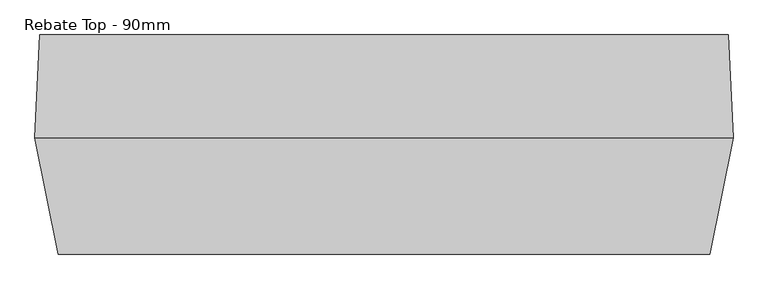
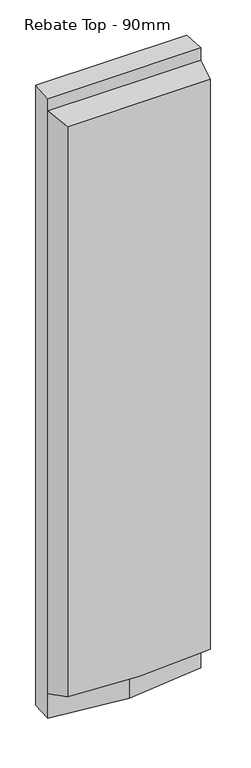
"""IFC4 building model written with IfcOpenShell, lengths in millimetres: proxy geometry, Industry_Buttress-Rebate_Top : Rebate Top - 90mm."""

from ifc_helpers import new_model, si_unit, origin, place, context, project, spatial, faceted_brep, source, transform, mapped, element, save


def rebate_top_90mm_773dfc1d(model_context):
    return source(origin(), model_context, "Body", "Brep", [
        faceted_brep([(-517.6, 155.0, 4530.0), (-525.0, 0.0, 4530.0), (525.0, 0.0, 4530.0), (517.6, 155.0, 4530.0), (-517.6, 155.0, 30.0), (517.6, 155.0, 30.0), (525.0, 0.0, 30.0), (0.0, -60.0, 30.0), (-525.0, 0.0, 30.0), (-525.0, 0.0, 210.0), (-525.0, 0.0, 4440.0), (-490.0, -175.0, 4420.0), (-490.0, -175.0, 283.2857143), (490.0, -175.0, 4420.0), (0.0, -175.0, 259.2857143), (490.0, -175.0, 283.2857143), (525.0, 0.0, 4440.0), (525.0, 0.0, 210.0), (0.0, -60.0, 210.0)], [[[0, 1, 2, 3]], [[4, 5, 6, 7, 8]], [[1, 0, 4, 8, 9, 10]], [[11, 10, 9, 12]], [[13, 11, 12, 14, 15]], [[16, 13, 15, 17]], [[3, 2, 16, 17, 6, 5]], [[0, 3, 5, 4]], [[16, 10, 11, 13]], [[10, 16, 2, 1]], [[18, 9, 8, 7]], [[9, 18, 14, 12]], [[17, 18, 7, 6]], [[18, 17, 15, 14]]]),
    ])


if __name__ == "__main__":
    model = new_model("IFC4")
    model_context = context("Model", 3, world=origin())
    ifc_project = project(units=[si_unit("LENGTHUNIT", "METRE", prefix="MILLI")], contexts=[model_context])
    site = spatial("IfcSite", under=ifc_project)
    building = spatial("IfcBuilding", under=site)
    placement = place(None, origin())
    rebate_top_90mm_shape = rebate_top_90mm_773dfc1d(model_context)
    element("IfcBuildingElementProxy", 1, Name="Industry_Buttress-Rebate_Top : Rebate Top - 90mm", ObjectType="Industry_Buttress-Rebate_Top : Rebate Top - 90mm", at=placement, inside=building, context=model_context, shape_type="MappedRepresentation", body=[
        mapped(rebate_top_90mm_shape, transform((0.0, 0.0, 0.0), x_axis=(1.0, 0.0, 0.0), y_axis=(0.0, 1.0, 0.0), z_axis=(0.0, 0.0, 1.0))),
    ])
    save(model, "model.ifc")

# Revit data of these elements
# Type "Industry_Buttress-Rebate_Top : Rebate Top - 90mm"
#   ACT_Wall_RebarGrade = "500"
#   ACT_Wall_PretensionTendon = "EN10138-3-Y1860"
#   ACT_Wall_PanelType [instance default] = ""
#   ACT_Wall_Number [instance default] = ""
#   ACT_Wall_Finish-Outside = "Steel Form"
#   ACT_Wall_Finish-Inside = "Steel Float Form"
#   ACT_Wall_ExposureClass = ""
#   ACT_Wall_EN-Standard = "EN 13369"
#   ACT_Wall_ConcreteClass = "C35/45"
#   Total Thickness [instance default] = 290 mm
#   Top Rebate Outside Height = 110 mm
#   Top Rebate Inside Height = 90 mm
#   Thickness [instance default] = 115 mm
#   Pitch [instance default] = 15 mm
#   Max Width = 1050 mm
#   Bottom Rebate Outside Height = 255 mm
#   Bottom Rebate Inside Height = 180 mm
#   ACT_Wall_Width [instance default] = 1050 mm
#   ACT_Wall_Height [instance default] = 4000 mm
#   Default Elevation = 0
# Element 1 (IfcBuildingElementProxy, "Industry_Buttress-Rebate_Top : Rebate Top - 90mm")
#   ACT_Wall_PanelType = "Buttress 01"
#   ACT_Wall_Number = "B2"
#   Total Thickness = 330 mm
#   Thickness = 155 mm
#   Pitch = 7.4 mm
#   ACT_Wall_Height = 4500 mm
#   Materials on its faces: "Concrete, Precast Smooth, Light Grey"
# Materials
#   "Concrete, Precast Smooth, Light Grey": class "Concrete", colour RGB 120 120 120, transparency 0, Description = "Precast concrete, light grey", Cost = 0
